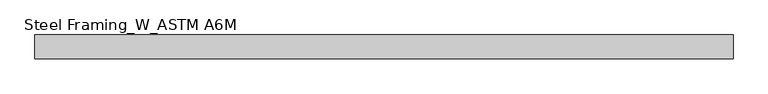
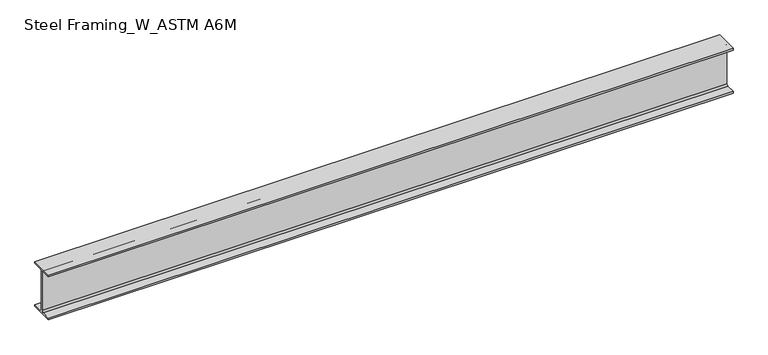
"""IFC4 building model written with IfcOpenShell, lengths in millimetres: beam geometry, Steel Framing_W_ASTM A6M : H_SB_AR_S02_W200x22.5_RB5."""

from ifc_helpers import new_model, si_unit, point, frame, frame_2d, origin, place, context, project, spatial, polyline, circle_curve, trimmed, segment, composite_curve, outline, extrude, source, transform, mapped, element, save


def steel_framing_w_astm_a6m_c4277c11(model_context):
    return source(origin(), model_context, "Body", "SweptSolid", [
        extrude(outline(composite_curve([segment(polyline([(51.0, -95.0), (51.0, -103.0), (-51.0, -103.0), (-51.0, -95.0), (-10.71, -95.0)]), True, "CONTINUOUS"), segment(trimmed(circle_curve(frame_2d((-10.71, -87.4)), 7.6), [point((-10.71, -95.0))], [point((-3.11, -87.4))], True, "CARTESIAN"), True, "CONTINUOUS"), segment(polyline([(-3.11, -87.4), (-3.11, 87.4)]), True, "CONTINUOUS"), segment(trimmed(circle_curve(frame_2d((-10.71, 87.4)), 7.6), [point((-3.11, 87.4))], [point((-10.71, 95.0))], True, "CARTESIAN"), True, "CONTINUOUS"), segment(polyline([(-10.71, 95.0), (-51.0, 95.0), (-51.0, 103.0), (51.0, 103.0), (51.0, 95.0), (10.71, 95.0)]), True, "CONTINUOUS"), segment(trimmed(circle_curve(frame_2d((10.71, 87.4)), 7.6), [point((10.71, 95.0))], [point((3.11, 87.4))], True, "CARTESIAN"), True, "CONTINUOUS"), segment(polyline([(3.11, 87.4), (3.11, -87.4)]), True, "CONTINUOUS"), segment(trimmed(circle_curve(frame_2d((10.71, -87.4)), 7.6), [point((3.11, -87.4))], [point((10.71, -95.0))], True, "CARTESIAN"), True, "CONTINUOUS"), segment(polyline([(10.71, -95.0), (51.0, -95.0)]), True, "CONTINUOUS")], self_intersect=False)), frame((-1487.2, 0.0, 0.0), z_axis=(1.0, 0.0, 0.0), x_axis=(0.0, 1.0, 0.0)), (0.0, 0.0, 1.0), 2974.4),
    ])


if __name__ == "__main__":
    model = new_model("IFC4")
    model_context = context("Model", 3, world=origin())
    ifc_project = project(units=[si_unit("LENGTHUNIT", "METRE", prefix="MILLI")], contexts=[model_context])
    site = spatial("IfcSite", under=ifc_project)
    building = spatial("IfcBuilding", under=site)
    placement = place(None, origin())
    steel_framing_w_astm_a6m_shape = steel_framing_w_astm_a6m_c4277c11(model_context)
    element("IfcBeam", 1, ObjectType="Steel Framing_W_ASTM A6M : H_SB_AR_S02_W200x22.5_RB5", at=placement, inside=building, context=model_context, shape_type="MappedRepresentation", body=[
        mapped(steel_framing_w_astm_a6m_shape, transform((0.0, 0.0, 0.0), x_axis=(1.0, 0.0, 0.0), y_axis=(0.0, 1.0, 0.0), z_axis=(0.0, 0.0, 1.0))),
    ])
    save(model, "model.ifc")

# Revit data of these elements
# Type "Steel Framing_W_ASTM A6M : H_SB_AR_S02_W200x22.5_RB5"
#   Type Mark = "RB5"
#   Section Name Key = "W8x15"
#   Width = 10.2 cm
#   Web Thickness = 0.622 cm
#   Web Fillet = 0.76 cm
#   Warping Constant = 13900.0 cm⁶
#   Torsional Moment of Inertia = 5.70 cm⁴
#   Section Area = 28.6 cm²
#   Plastic Modulus weak axis = 43.8 cm³
#   Plastic Modulus strong axis = 223.0 cm³
#   Perimeter = 0.795 m²/m
#   Nominal Weight = 22.50 kgf/m
#   Moment of Inertia weak axis = 142.00 cm⁴
#   Moment of Inertia strong axis = 2000.00 cm⁴
#   Height = 20.6 cm
#   Flange Thickness = 0.8 cm
#   Elastic Modulus weak axis = 27.9 cm³
#   Elastic Modulus strong axis = 193.0 cm³
#   Centroid Vertical = 10.3 cm
#   Centroid Horizontal = 5.1 cm
#   Length [instance default] = 1500 mm
#   Structural Material [instance default] = Steel, 45-345
#   Bolt Spacing = 0
#   Assembly Code = ""
# Element 1 (IfcBeam, "Steel Framing_W_ASTM A6M : H_SB_AR_S02_W200x22.5_RB5")
#   Materials on its faces: "Steel, 45-345"
# Materials
#   "Steel, 45-345": class "Metal", colour RGB 189 187 185, transparency 0, Description = "Steel 345 MPa", Cost = 0
